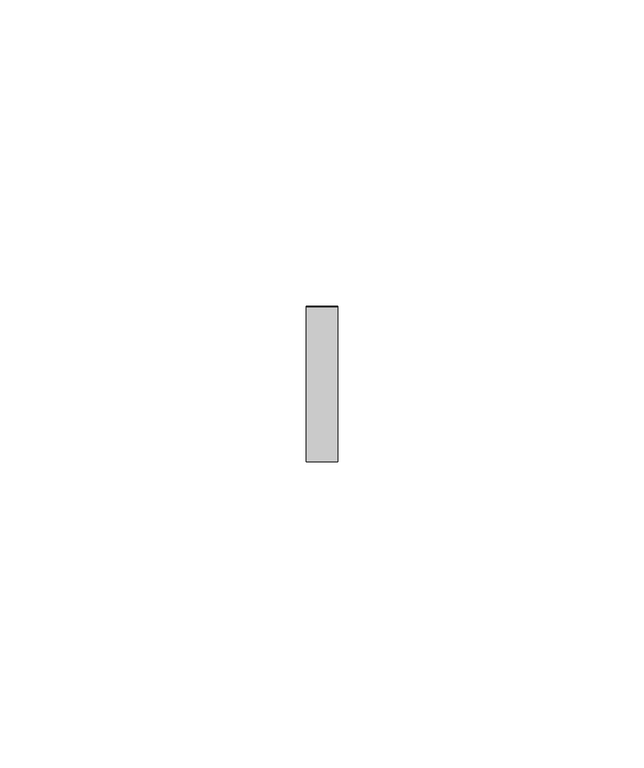
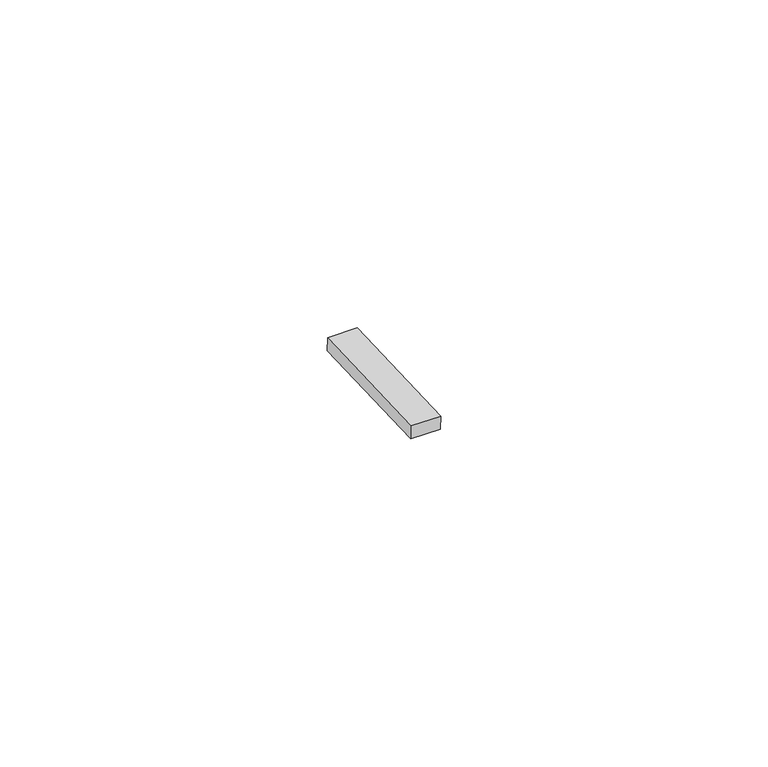
"""IFC4 building model written with IfcOpenShell, lengths in millimetres: proxy geometry, Inner panel:Inner panel:1:Inner panel:1 : Inner panel:Inner panel:300324:2:Inner panel:1:Inner panel:1 : Inner panel:Inner panel:300324:2 : Inner panel:Inner panel:1:Inner panel:1 : Inner panel:Inner panel:300324:300043:6 : Inner panel:Inner panel:1:Inner panel:1 : Inner panel:Inner panel:300324:2:Inner panel:1:Inner panel:1 : Inner panel:Inner panel:300324:2 : Inner panel:Inner panel:1:Inner panel:1 : Inner panel:Inner panel:300324:300043:308120."""

from ifc_helpers import new_model, si_unit, frame, origin, place, context, project, spatial, polyline, outline, extrude, source, transform, mapped, element, save


def generic_models_75057a99(model_context):
    return source(origin(), model_context, "Body", "SweptSolid", [
        extrude(outline(polyline([(0.0, -25.3999999), (0.0, 0.0), (5.2138089, 0.0), (5.2138089, -25.3999999), (0.0, -25.3999999)])), frame((593530.195117, -569673.6314539, 8741.7380349), z_axis=(0.0, -0.041630544712223896, 0.9991330730923502), x_axis=(-1.0, 0.0, 0.0)), (0.0, 0.0, 1.0), 2.4763745),
    ])


if __name__ == "__main__":
    model = new_model("IFC4")
    model_context = context("Model", 3, world=origin())
    ifc_project = project(units=[si_unit("LENGTHUNIT", "METRE", prefix="MILLI")], contexts=[model_context])
    site = spatial("IfcSite", under=ifc_project)
    building = spatial("IfcBuilding", under=site)
    placement = place(None, origin())
    generic_models_shape = generic_models_75057a99(model_context)
    element("IfcBuildingElementProxy", 1, Name="Inner panel:Inner panel:1:Inner panel:1 : Inner panel:Inner panel:300324:2:Inner panel:1:Inner panel:1 : Inner panel:Inner panel:300324:2 : Inner panel:Inner panel:1:Inner panel:1 : Inner panel:Inner panel:300324:300043:6 : Inner panel:Inner panel:1:Inner panel:1 : Inner panel:Inner panel:300324:2:Inner panel:1:Inner panel:1 : Inner panel:Inner panel:300324:2 : Inner panel:Inner panel:1:Inner panel:1 : Inner panel:Inner panel:300324:300043:308120", ObjectType="Inner panel:Inner panel:1:Inner panel:1 : Inner panel:Inner panel:300324:2:Inner panel:1:Inner panel:1 : Inner panel:Inner panel:300324:2 : Inner panel:Inner panel:1:Inner panel:1 : Inner panel:Inner panel:300324:300043:6 : Inner panel:Inner panel:1:Inner panel:1 : Inner panel:Inner panel:300324:2:Inner panel:1:Inner panel:1 : Inner panel:Inner panel:300324:2 : Inner panel:Inner panel:1:Inner panel:1 : Inner panel:Inner panel:300324:300043:308120", at=placement, inside=building, context=model_context, shape_type="MappedRepresentation", body=[
        mapped(generic_models_shape, transform((0.0, 0.0, 0.0), x_axis=(1.0, 0.0, 0.0), y_axis=(0.0, 1.0, 0.0), z_axis=(0.0, 0.0, 1.0))),
    ])
    save(model, "model.ifc")

# Revit data of these elements
# Type "Inner panel:Inner panel:1:Inner panel:1 : Inner panel:Inner panel:300324:2:Inner panel:1:Inner panel:1 : Inner panel:Inner panel:300324:2 : Inner panel:Inner panel:1:Inner panel:1 : Inner panel:Inner panel:300324:300043:6 : Inner panel:Inner panel:1:Inner panel:1 : Inner panel:Inner panel:300324:2:Inner panel:1:Inner panel:1 : Inner panel:Inner panel:300324:2 : Inner panel:Inner panel:1:Inner panel:1 : Inner panel:Inner panel:300324:300043:308120"
#   NameOverride = "Inner panel:Inner panel:1:Inner panel:1 : Inner panel:Inner panel:300324:2:Inner panel:1:Inner panel:1 : Inner panel:Inner panel:300324:2 : Inner panel:Inner panel:1:Inner panel:1 : Inner panel:Inner panel:300324:300043:308120"
#   ObjectTypeOverride = "Inner panel:1:Inner panel:1 : Inner panel:Inner panel:300324:2 : Inner panel:Inner panel:1:Inner panel:1 : Inner panel:Inner panel:300324:300043"
#   Reference = "Inner panel"
#   Tag = "308120"
# Element 1 (IfcBuildingElementProxy, "Inner panel:Inner panel:1:Inner panel:1 : Inner panel:Inner panel:300324:2:Inner panel:1:Inner panel:1 : Inner panel:Inner panel:300324:2 : Inner panel:Inner panel:1:Inner panel:1 : Inner panel:Inner panel:300324:300043:6 : Inner panel:Inner panel:1:Inner panel:1 : Inner panel:Inner panel:300324:2:Inner panel:1:Inner panel:1 : Inner panel:Inner panel:300324:2 : Inner panel:Inner panel:1:Inner panel:1 : Inner panel:Inner panel:300324:300043:308120")
#   Materials on its faces: "AT CLIP - 1\" WIDE NON ABSORBENT, WEATHER-RESISTANT NEOPRENE/EPDM/SBR FOAM"
# Materials
#   "AT CLIP - 1\" WIDE NON ABSORBENT, WEATHER-RESISTANT NEOPRENE/EPDM/SBR FOAM": class "Generic", colour RGB 85 85 85, transparency 0, Cost = 0
